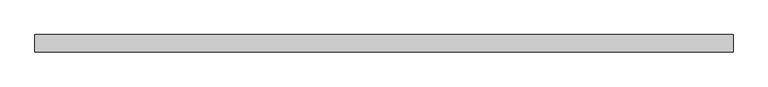
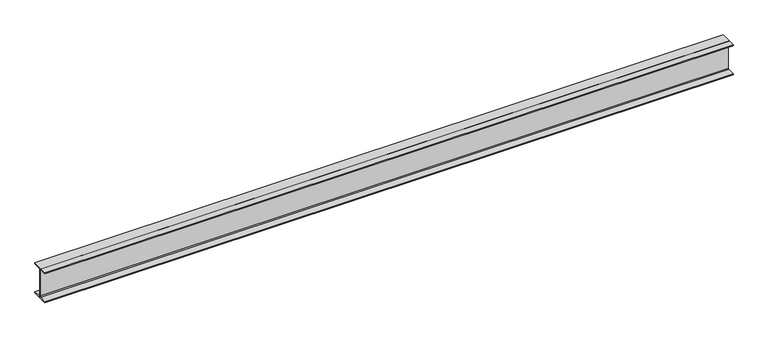
"""IFC4 building model written with IfcOpenShell, lengths in millimetres: beam geometry, Old_Steel Beam_H-KSD3502 : H_SB_ASB_H-350×175x7x11."""

from ifc_helpers import new_model, si_unit, point, frame, frame_2d, origin, place, context, project, spatial, polyline, circle_curve, trimmed, segment, composite_curve, outline, extrude, source, transform, mapped, element, save


def beam_245fb9f8(model_context):
    return source(origin(), model_context, "Body", "SweptSolid", [
        extrude(outline(composite_curve([segment(polyline([(82.5, -141.5), (82.5, -151.7), (-82.5, -151.7), (-82.5, -141.5), (-11.9, -141.5)]), True, "CONTINUOUS"), segment(trimmed(circle_curve(frame_2d((-11.9, -132.6)), 8.9), [point((-11.9, -141.5))], [point((-3.0, -132.6))], True, "CARTESIAN"), True, "CONTINUOUS"), segment(polyline([(-3.0, -132.6), (-3.0, 132.6)]), True, "CONTINUOUS"), segment(trimmed(circle_curve(frame_2d((-11.9, 132.6)), 8.9), [point((-3.0, 132.6))], [point((-11.9, 141.5))], True, "CARTESIAN"), True, "CONTINUOUS"), segment(polyline([(-11.9, 141.5), (-82.5, 141.5), (-82.5, 151.7), (82.5, 151.7), (82.5, 141.5), (11.9, 141.5)]), True, "CONTINUOUS"), segment(trimmed(circle_curve(frame_2d((11.9, 132.6)), 8.9), [point((11.9, 141.5))], [point((3.0, 132.6))], True, "CARTESIAN"), True, "CONTINUOUS"), segment(polyline([(3.0, 132.6), (3.0, -132.6)]), True, "CONTINUOUS"), segment(trimmed(circle_curve(frame_2d((11.9, -132.6)), 8.9), [point((3.0, -132.6))], [point((11.9, -141.5))], True, "CARTESIAN"), True, "CONTINUOUS"), segment(polyline([(11.9, -141.5), (82.5, -141.5)]), True, "CONTINUOUS")], self_intersect=False)), frame((-3262.3, 0.0, 0.0), z_axis=(1.0, 0.0, 0.0), x_axis=(0.0, 1.0, 0.0)), (0.0, 0.0, 1.0), 6599.6),
    ])


if __name__ == "__main__":
    model = new_model("IFC4")
    model_context = context("Model", 3, world=origin())
    ifc_project = project(units=[si_unit("LENGTHUNIT", "METRE", prefix="MILLI")], contexts=[model_context])
    site = spatial("IfcSite", under=ifc_project)
    building = spatial("IfcBuilding", under=site)
    placement = place(None, origin())
    beam_shape = beam_245fb9f8(model_context)
    element("IfcBeam", 1, ObjectType="Old_Steel Beam_H-KSD3502 : H_SB_ASB_H-350×175x7x11", at=placement, inside=building, context=model_context, shape_type="MappedRepresentation", body=[
        mapped(beam_shape, transform((0.0, 0.0, 0.0), x_axis=(1.0, 0.0, 0.0), y_axis=(0.0, 1.0, 0.0), z_axis=(0.0, 0.0, 1.0))),
    ])
    save(model, "model.ifc")

# Revit data of these elements
# Type "Old_Steel Beam_H-KSD3502 : H_SB_ASB_H-350×175x7x11"
#   Width = 17.5 cm
#   Web Thickness = 0.7 cm
#   Web Fillet = 1.4 cm
#   Warping Constant = 282290.0 cm⁶
#   Torsional Moment of Inertia = 19.4042 cm⁴
#   Torsional Modulus = 1.0 cm³
#   Section Area = 63.14 cm²
#   Plastic Modulus weak axis = 174.0 cm³
#   Plastic Modulus strong axis = 868.0 cm³
#   Perimeter = 1.36 m²/m
#   Nominal Weight = 49.60 kgf/m
#   Moment of Inertia weak axis = 984.00 cm⁴
#   Moment of Inertia strong axis = 13600.00 cm⁴
#   Height = 35.0 cm
#   Flange Thickness = 1.1 cm
#   Elastic Modulus weak axis = 112.0 cm³
#   Elastic Modulus strong axis = 775.0 cm³
#   Centroid Vertical = 17.5 cm
#   Centroid Horizontal = 8.75 cm
#   Length [instance default] = 1.5240 m
#   Structural Material [instance default] = Steel, 45-345
#   Assembly Code = ""
# Element 1 (IfcBeam, "Old_Steel Beam_H-KSD3502 : H_SB_ASB_H-350×175x7x11")
#   Structural Material = none
# Materials
#   "Steel, 45-345": class "Metal", colour RGB 189 187 185, transparency 0, Description = "Steel 345 MPa", Cost = 0
